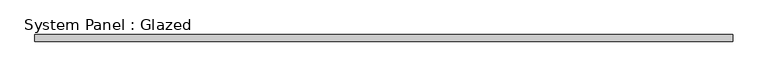
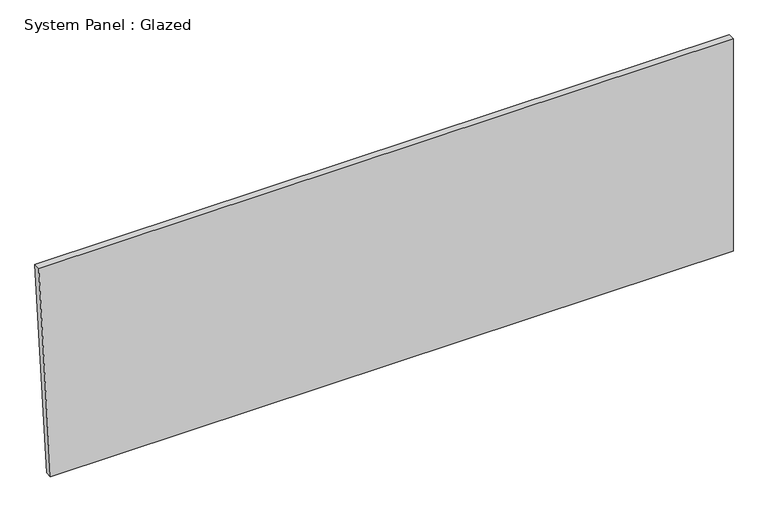
"""IFC4 building model written with IfcOpenShell, lengths in millimetres: plate geometry, System Panel : Glazed."""

import ifcopenshell
import ifcopenshell.guid

model = None  # the IFC model being written
_history = None  # IfcOwnerHistory: only IFC2X3 demands one
_inside = {}  # id of a spatial element -> (the spatial element, [elements in it])
_under = {}  # id of a project, library or spatial element -> (it, [spatial elements below it])
_declared = {}  # id of a project -> (the project, [libraries it declares])
_typed = {}  # id of a type object -> (the type object, [elements of that type])
_made_of = {}  # id of a material, layer set ... -> (it, [elements and type objects made of it])


def new_model(schema):
    """Start an empty IFC model of exactly this schema.

    Asked for "IFC4X3", IfcOpenShell would pick the latest addendum, in which some entities
    have other attributes; the version numbers below select the first issue.
    IFC2X3 requires an IfcOwnerHistory on every rooted entity: one is made here for all.
    """
    global model, _history
    if schema == "IFC4X3":
        model = ifcopenshell.file(schema_version=(4, 3, 0, 0))
    else:
        model = ifcopenshell.file(schema=schema)
    _inside.clear()
    _under.clear()
    _declared.clear()
    _typed.clear()
    _made_of.clear()
    _history = None
    if model.schema == "IFC2X3":
        org = make("IfcOrganization", Name="unknown")
        user = make(
            "IfcPersonAndOrganization",
            ThePerson=make("IfcPerson", FamilyName="unknown"),
            TheOrganization=org,
        )
        app = make(
            "IfcApplication",
            ApplicationDeveloper=org,
            Version="unknown",
            ApplicationFullName="unknown",
            ApplicationIdentifier="unknown",
        )
        _history = make(
            "IfcOwnerHistory",
            OwningUser=user,
            OwningApplication=app,
            ChangeAction="ADDED",
            CreationDate=0,
        )
    return model


def make(cls, **values):
    """One entity of the class cls with the attributes given. An attribute that is None is left unset."""
    return model.create_entity(
        cls, **{name: value for name, value in values.items() if value is not None}
    )


def rooted(cls, **values):
    """An entity with a GlobalId (a new one), such as an element, a storey or a relation."""
    return make(cls, GlobalId=ifcopenshell.guid.new(), OwnerHistory=_history, **values)


def si_unit(unit_type, name, prefix=None):
    """IfcSIUnit, for example si_unit("LENGTHUNIT", "METRE", prefix="MILLI")."""
    return make("IfcSIUnit", UnitType=unit_type, Prefix=prefix, Name=name)


def assignment(units):
    """IfcUnitAssignment: the units of a project."""
    return None if units is None else make("IfcUnitAssignment", Units=units)


def point(xyz):
    """IfcCartesianPoint."""
    return None if xyz is None else make("IfcCartesianPoint", Coordinates=xyz)


def direction(xyz):
    """IfcDirection."""
    return None if xyz is None else make("IfcDirection", DirectionRatios=xyz)


def frame(location, z_axis=None, x_axis=None):
    """IfcAxis2Placement3D, a coordinate frame: its origin and axes. An axis left out is left unset."""
    return make(
        "IfcAxis2Placement3D",
        Location=point(location),
        Axis=direction(z_axis),
        RefDirection=direction(x_axis),
    )


def origin():
    """The frame at (0, 0, 0) with its axes left unset."""
    return frame((0.0, 0.0, 0.0))


def place(relative_to, where):
    """IfcLocalPlacement: puts the frame where relative to a parent placement (None: the world)."""
    return make(
        "IfcLocalPlacement", PlacementRelTo=relative_to, RelativePlacement=where
    )


def context(
    kind, dimensions, precision=None, world=None, true_north=None, identifier=None
):
    """IfcGeometricRepresentationContext, for example the 3D "Model" context."""
    return make(
        "IfcGeometricRepresentationContext",
        ContextIdentifier=identifier,
        ContextType=kind,
        CoordinateSpaceDimension=dimensions,
        Precision=precision,
        WorldCoordinateSystem=world,
        TrueNorth=true_north,
    )


def project(units=None, contexts=None):
    """IfcProject with its units and contexts."""
    return rooted(
        "IfcProject",
        Name="project",
        RepresentationContexts=contexts,
        UnitsInContext=assignment(units),
    )


def spatial(cls, under=None, at=None, **own):
    """A site, building, storey or space (cls), placed at a placement, below another one or the project."""
    s = rooted(cls, ObjectPlacement=at, **own)
    if under is not None:
        _under.setdefault(under.id(), (under, []))[1].append(s)
    return s


def polyline(points):
    """IfcPolyline through the points."""
    return make("IfcPolyline", Points=[point(p) for p in points])


def outline(outer, holes=None, kind="AREA"):
    """IfcArbitraryClosedProfileDef: a profile drawn as a closed curve; with holes, ...WithVoids."""
    if holes is None:
        return make("IfcArbitraryClosedProfileDef", ProfileType=kind, OuterCurve=outer)
    return make(
        "IfcArbitraryProfileDefWithVoids",
        ProfileType=kind,
        OuterCurve=outer,
        InnerCurves=holes,
    )


def extrude(swept, where, along, depth):
    """IfcExtrudedAreaSolid: the profile swept, set in the frame where, extruded along a direction by depth."""
    return make(
        "IfcExtrudedAreaSolid",
        SweptArea=swept,
        Position=where,
        ExtrudedDirection=direction(along),
        Depth=depth,
    )


def shape(context_of_items, identifier, shape_type, items):
    """IfcShapeRepresentation: the items that make up one representation, for example the "Body"."""
    return make(
        "IfcShapeRepresentation",
        ContextOfItems=context_of_items,
        RepresentationIdentifier=identifier,
        RepresentationType=shape_type,
        Items=items,
    )


def source(mapping_origin, context_of_items, identifier, shape_type, items):
    """IfcRepresentationMap: a shape defined once, which mapped items show again and again."""
    return make(
        "IfcRepresentationMap",
        MappingOrigin=mapping_origin,
        MappedRepresentation=shape(context_of_items, identifier, shape_type, items),
    )


def transform(
    local_origin,
    x_axis=None,
    y_axis=None,
    z_axis=None,
    scale=None,
    scale2=None,
    scale3=None,
    uniform=True,
):
    """IfcCartesianTransformationOperator3D, or its non-uniform kind. x_axis, y_axis, z_axis: its Axis1, 2, 3."""
    if uniform:
        return make(
            "IfcCartesianTransformationOperator3D",
            Axis1=direction(x_axis),
            Axis2=direction(y_axis),
            LocalOrigin=point(local_origin),
            Scale=scale,
            Axis3=direction(z_axis),
        )
    return make(
        "IfcCartesianTransformationOperator3DnonUniform",
        Axis1=direction(x_axis),
        Axis2=direction(y_axis),
        LocalOrigin=point(local_origin),
        Scale=scale,
        Axis3=direction(z_axis),
        Scale2=scale2,
        Scale3=scale3,
    )


def mapped(mapping_source, mapping_target):
    """IfcMappedItem: shows the shape of a source again, moved by a transform."""
    return make(
        "IfcMappedItem", MappingSource=mapping_source, MappingTarget=mapping_target
    )


def made_of(thing, what):
    """Note that an element or type object is made of a material, layer set ...; save() writes the relation."""
    if what is not None:
        _made_of.setdefault(what.id(), (what, []))[1].append(thing)
    return thing


def element(
    cls,
    number,
    at=None,
    inside=None,
    cuts=None,
    type_object=None,
    material=None,
    context=None,
    identifier="Body",
    shape_type=None,
    held_by="IfcProductDefinitionShape",
    body=None,
    shapes=None,
    **own,
):
    """One element of the class cls, such as IfcWall. Its Tag is "e" and its number.

    at: its placement. inside: the storey or other place that contains it. cuts: it is an
    opening in that element (IfcRelVoidsElement). A single representation is given by context,
    identifier, shape_type and body (its items); several are given by shapes. held_by: the class
    of the entity that holds the representations. save() writes the other relations.
    """
    e = rooted(cls, Tag="e%d" % number, ObjectPlacement=at, **own)
    if body is not None:
        shapes = [shape(context, identifier, shape_type, body)]
    if shapes is not None:
        e.Representation = make(held_by, Representations=shapes)
    if inside is not None:
        _inside.setdefault(inside.id(), (inside, []))[1].append(e)
    if cuts is not None:
        rooted(
            "IfcRelVoidsElement", RelatingBuildingElement=cuts, RelatedOpeningElement=e
        )
    if type_object is not None:
        _typed.setdefault(type_object.id(), (type_object, []))[1].append(e)
    return made_of(e, material)


def aggregate(whole, parts):
    """IfcRelAggregates: a whole, such as a stair, and the parts it consists of."""
    return rooted("IfcRelAggregates", RelatingObject=whole, RelatedObjects=parts)


def save(model, path):
    """Write the relations noted so far, then the file.

    IfcRelAggregates (storeys below a building ...), IfcRelContainedInSpatialStructure (elements
    in a storey), IfcRelDefinesByType, IfcRelAssociatesMaterial and IfcRelDeclares: one each for
    every whole, place, type object, material and project.
    """
    for whole, parts in _under.values():
        aggregate(whole, parts)
    for where, things in _inside.values():
        rooted(
            "IfcRelContainedInSpatialStructure",
            RelatedElements=things,
            RelatingStructure=where,
        )
    for kind, things in _typed.values():
        rooted("IfcRelDefinesByType", RelatedObjects=things, RelatingType=kind)
    for what, things in _made_of.values():
        rooted("IfcRelAssociatesMaterial", RelatedObjects=things, RelatingMaterial=what)
    for by, libraries in _declared.values():
        rooted("IfcRelDeclares", RelatingContext=by, RelatedDefinitions=libraries)
    model.write(path)


def system_panel_glazed_52faa4d2(model_context):
    return source(origin(), model_context, "Body", "SweptSolid", [
        extrude(outline(polyline([(0.0, -1293.230316), (0.0, 1338.5575225), (866.081558, 1338.5575225), (866.081558, -1338.5575225), (0.0, -1293.230316)])), frame((0.0, -44.45, 0.0), z_axis=(0.0, 1.0, 0.0), x_axis=(0.0, 0.0, 1.0)), (0.0, 0.0, 1.0), 25.4),
    ])


if __name__ == "__main__":
    model = new_model("IFC4")
    model_context = context("Model", 3, world=origin())
    ifc_project = project(units=[si_unit("LENGTHUNIT", "METRE", prefix="MILLI")], contexts=[model_context])
    site = spatial("IfcSite", under=ifc_project)
    building = spatial("IfcBuilding", under=site)
    placement = place(None, origin())
    system_panel_glazed_shape = system_panel_glazed_52faa4d2(model_context)
    element("IfcPlate", 1, ObjectType="System Panel : Glazed", at=placement, inside=building, context=model_context, shape_type="MappedRepresentation", body=[
        mapped(system_panel_glazed_shape, transform((0.0, 0.0, 0.0), x_axis=(1.0, 0.0, 0.0), y_axis=(0.0, 1.0, 0.0), z_axis=(0.0, 0.0, 1.0))),
    ])
    save(model, "model.ifc")

# Revit data of these elements
# Type "System Panel : Glazed"
#   Construction Type Id = "GSP4R"
#   Analytic Construction = "1/8 in Pilkington single glazing"
#   Visual Light Transmittance = 0.9
#   Solar Heat Gain Coefficient = 0.86
#   Heat Transfer Coefficient (U) = 1.18115 BTU/(h·ft²·°F)
#   Define Thermal Properties by = 1
# Element 1 (IfcPlate, "System Panel : Glazed")
#   Materials on its faces: "Glass"
# Materials
#   "Glass": class "Glass", colour RGB 0 128 192, transparency 0.75, Description = "Soda Lime Glass", Cost = 0
